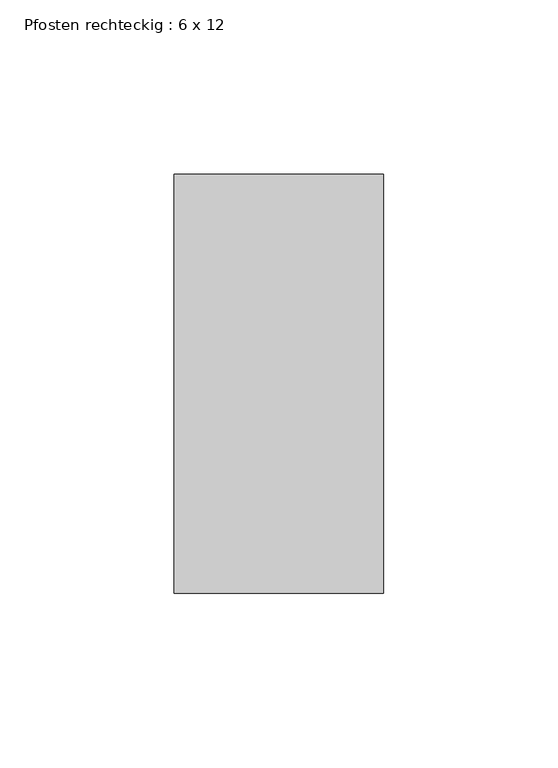
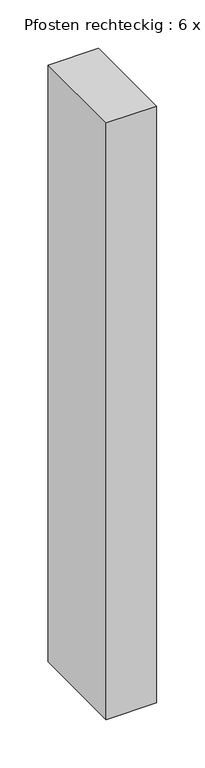
"""IFC4 building model written with IfcOpenShell, lengths in millimetres: member geometry, Pfosten rechteckig : 6 x 12."""

from ifc_helpers import new_model, si_unit, frame, origin, place, context, project, spatial, polyline, outline, extrude, source, transform, mapped, element, save


def pfosten_rechteckig_6_x_12_3d8c6ebc(model_context):
    return source(origin(), model_context, "Body", "SweptSolid", [
        extrude(outline(polyline([(30.0, 60.0), (30.0, -60.0), (-30.0, -60.0), (-30.0, 60.0), (30.0, 60.0)])), frame((0.0, 0.0, -752.9462629), z_axis=(0.0, 0.0, 1.0), x_axis=(1.0, 0.0, 0.0)), (0.0, 0.0, 1.0), 752.9462629),
    ])


if __name__ == "__main__":
    model = new_model("IFC4")
    model_context = context("Model", 3, world=origin())
    ifc_project = project(units=[si_unit("LENGTHUNIT", "METRE", prefix="MILLI")], contexts=[model_context])
    site = spatial("IfcSite", under=ifc_project)
    building = spatial("IfcBuilding", under=site)
    placement = place(None, origin())
    pfosten_rechteckig_6_x_12_shape = pfosten_rechteckig_6_x_12_3d8c6ebc(model_context)
    element("IfcMember", 1, ObjectType="Pfosten rechteckig : 6 x 12", at=placement, inside=building, context=model_context, shape_type="MappedRepresentation", body=[
        mapped(pfosten_rechteckig_6_x_12_shape, transform((0.0, 0.0, 0.0), x_axis=(1.0, 0.0, 0.0), y_axis=(0.0, 1.0, 0.0), z_axis=(0.0, 0.0, 1.0))),
    ])
    save(model, "model.ifc")

# Revit data of these elements
# Type "Pfosten rechteckig : 6 x 12"
#   built-in parameter 1007304 = 0.393701 (stored number, unit not read)
#   built-in parameter 1007301 = 0.0984252 (stored number, unit not read)
#   built-in parameter 1007300 = 0.0984252 (stored number, unit not read)
# Element 1 (IfcMember, "Pfosten rechteckig : 6 x 12")
#   Materials on its faces: "Metall - verzinkt"
# Materials
#   "Metall - verzinkt": class "Allgemeines", colour RGB 200 200 200, transparency 0, Cost = 0
